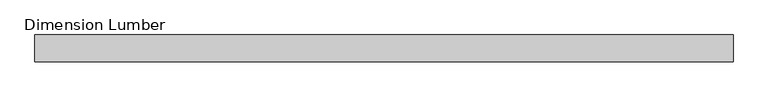
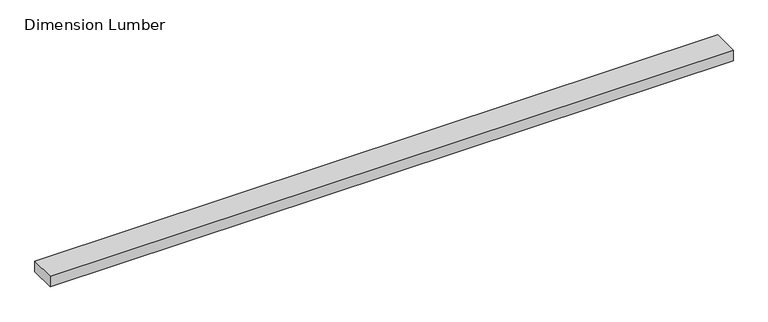
"""IFC4 building model written with IfcOpenShell, lengths in millimetres: beam geometry, Dimension Lumber : Top Supporting Lumbers."""

from ifc_helpers import new_model, si_unit, frame, origin, place, context, project, spatial, polyline, outline, extrude, source, transform, mapped, element, save


def dimension_lumber_bb8f2985(model_context):
    return source(origin(), model_context, "Body", "SweptSolid", [
        extrude(outline(polyline([(1149.3500003, 44.45), (1149.3500003, -44.45), (-1149.3500003, -44.45), (-1149.3500003, 44.45), (1149.3500003, 44.45)])), frame((0.0, 0.0, -19.05), z_axis=(0.0, 0.0, 1.0), x_axis=(1.0, 0.0, 0.0)), (0.0, 0.0, 1.0), 38.1),
    ])


if __name__ == "__main__":
    model = new_model("IFC4")
    model_context = context("Model", 3, world=origin())
    ifc_project = project(units=[si_unit("LENGTHUNIT", "METRE", prefix="MILLI")], contexts=[model_context])
    site = spatial("IfcSite", under=ifc_project)
    building = spatial("IfcBuilding", under=site)
    placement = place(None, origin())
    dimension_lumber_shape = dimension_lumber_bb8f2985(model_context)
    element("IfcBeam", 1, ObjectType="Dimension Lumber : Top Supporting Lumbers", at=placement, inside=building, context=model_context, shape_type="MappedRepresentation", body=[
        mapped(dimension_lumber_shape, transform((0.0, 0.0, 0.0), x_axis=(1.0, 0.0, 0.0), y_axis=(0.0, 1.0, 0.0), z_axis=(0.0, 0.0, 1.0))),
    ])
    save(model, "model.ifc")

# Revit data of these elements
# Type "Dimension Lumber : Top Supporting Lumbers"
#   Assembly Code = "B10"
#   A = 0.0364583 SF
#   Length [instance default] = 5' - 0"
#   b = 0' - 3 1/2"
#   d = 0' - 1 1/2"
#   Structural Material [instance default] = Softwood, Lumber
# Element 1 (IfcBeam, "Dimension Lumber : Top Supporting Lumbers")
#   Structural Material = Douglas Fir #2
#   Materials on its faces: "Douglas Fir #2"
# Materials
#   "Softwood, Lumber": class "Wood", colour RGB 223 192 134, transparency 0, Description = "Pinus Echinata", Cost = 0
#   "Douglas Fir #2": class "Wood", colour RGB 223 192 134, transparency 0, Description = "Pinus Echinata", Cost = 0
